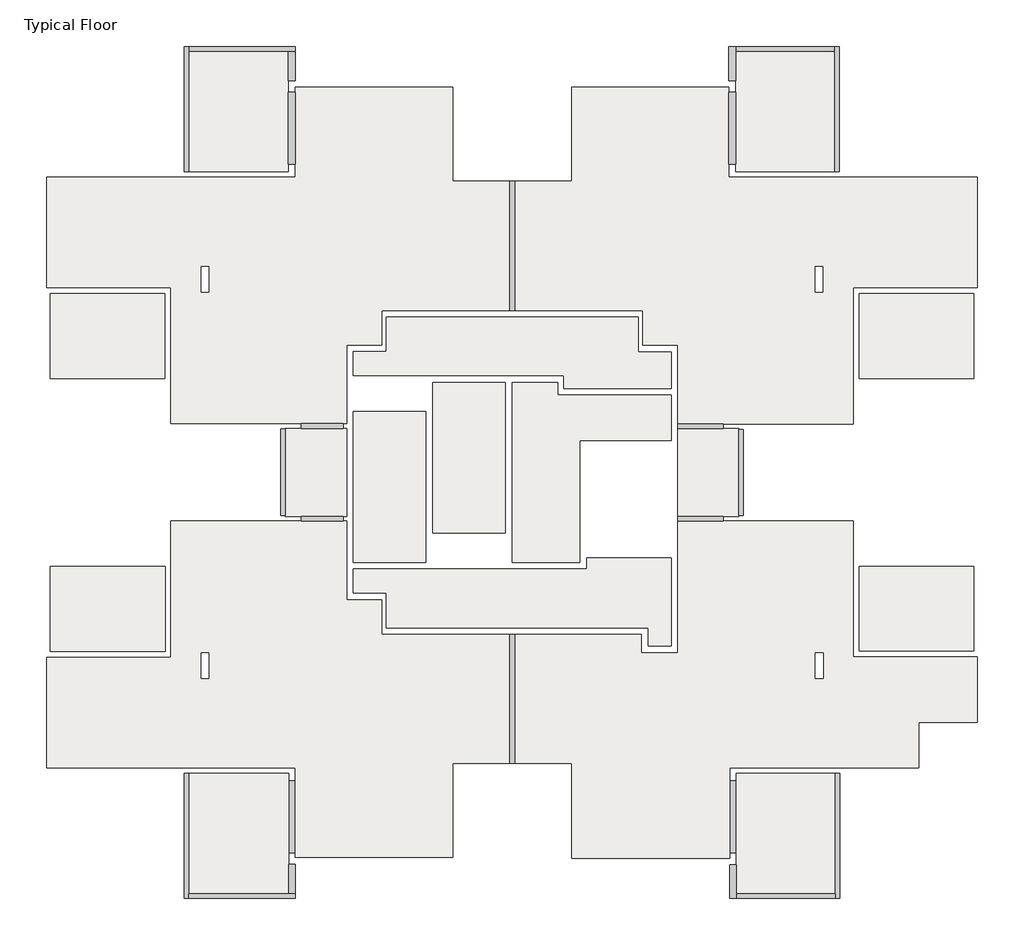
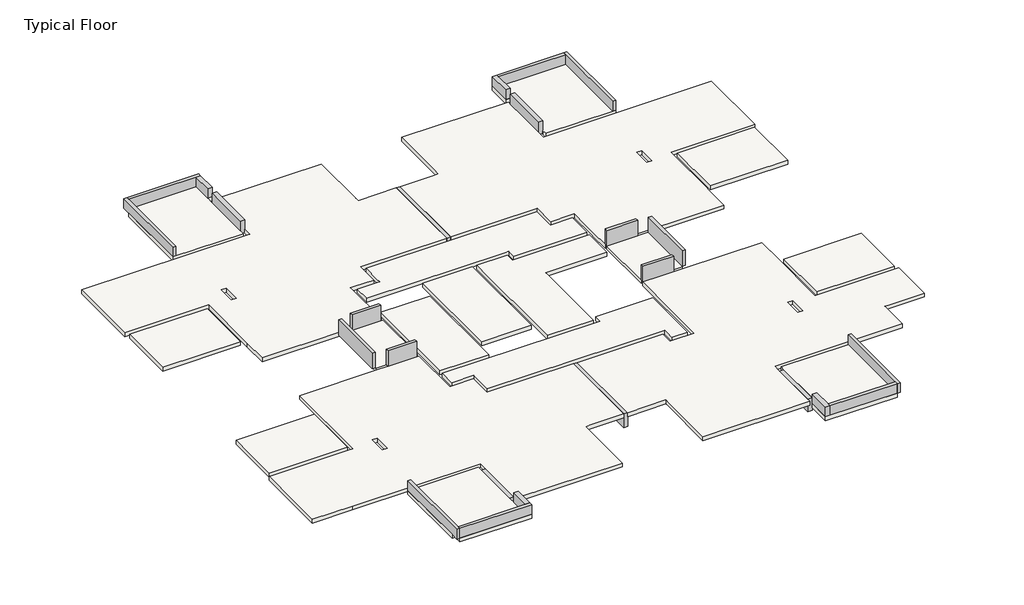
# One storey: 24 beams, 19 slabs.
"""IFC4 building model written with IfcOpenShell, lengths in millimetres."""

from ifc_helpers import new_model, si_unit, frame, origin, place, context, project, spatial, polyline, outline, extrude, faceted_brep, element, save

model = new_model("IFC4")

# Units and contexts
model_context = context("Model", 3, world=origin())
ifc_project = project(units=[si_unit("LENGTHUNIT", "METRE", prefix="MILLI")], contexts=[model_context])

# Site, building, storey
site = spatial("IfcSite", under=ifc_project)
building = spatial("IfcBuilding", under=site)
storey = spatial("IfcBuildingStorey", under=building, Name="Typical Floor", Elevation=3070.0)

# Beams
placement = place(None, origin())
element("IfcBeam", 1, ObjectType="Concrete Rectengular Beam : 15/50", at=placement, inside=storey, context=model_context, shape_type="Brep", body=[
    faceted_brep([(-14463.9862657, -10993.4504981, 3570.0), (-14313.9862657, -10993.4504981, 3570.0), (-14313.9862657, -10993.4504981, 3070.0), (-14463.9862657, -10993.4504981, 3070.0), (-14463.9862657, -15120.0113915, 3570.0), (-14313.9862657, -15120.0113915, 3570.0), (-14313.9862657, -14970.0113915, 3570.0), (-14313.9862657, -15120.0113915, 3070.0), (-14313.9862657, -14970.0113915, 3070.0), (-14313.9862657, -14720.0113915, 3070.0), (-14463.9862657, -15120.0113915, 3070.0), (-14463.9862657, -14720.0113915, 3070.0)], [[[0, 1, 2, 3]], [[1, 0, 4, 5, 6]], [[2, 1, 6, 5, 7, 8, 9]], [[3, 2, 9, 8, 7, 10, 11]], [[0, 3, 11, 10, 4]], [[5, 4, 10, 7]]]),
])
element("IfcBeam", 2, ObjectType="Concrete Rectengular Beam : 15/50", at=placement, inside=storey, context=model_context, shape_type="Brep", body=[
    faceted_brep([(-10809.6404044, -15120.0113915, 3570.0), (-10809.6404044, -14970.0113915, 3570.0), (-11029.6404044, -14970.0113915, 3570.0), (-14313.9862657, -14970.0113915, 3570.0), (-14313.9862657, -15120.0113915, 3570.0), (-10809.6404044, -15120.0113915, 3070.0), (-14313.9862657, -15120.0113915, 3070.0), (-10809.6404044, -14970.0113915, 3070.0), (-14313.9862657, -14970.0113915, 3070.0), (-11029.6404044, -14970.0113915, 3070.0)], [[[0, 1, 2, 3, 4]], [[5, 0, 4, 6]], [[7, 5, 6, 8, 9]], [[1, 7, 9, 8, 3, 2]], [[1, 0, 5, 7]], [[4, 3, 8, 6]]]),
])
element("IfcBeam", 3, ObjectType="Concrete Rectengular Beam : 15/50", at=placement, inside=storey, context=model_context, shape_type="Brep", body=[
    faceted_brep([(7011.4479352, -10993.4467583, 3570.0), (7161.4479352, -10993.4467583, 3570.0), (7161.4479352, -10993.4467583, 3070.0), (7011.4479352, -10993.4467583, 3070.0), (7011.4479352, -14970.0113915, 3570.0), (7011.4479352, -15120.0113915, 3570.0), (7161.4479352, -15120.0113915, 3570.0), (7011.4479352, -14720.0113915, 3070.0), (7011.4479352, -14970.0113915, 3070.0), (7011.4479352, -15120.0113915, 3070.0), (7161.4479352, -14720.0113915, 3070.0), (7161.4479352, -15120.0113915, 3070.0)], [[[0, 1, 2, 3]], [[1, 0, 4, 5, 6]], [[0, 3, 7, 8, 9, 5, 4]], [[3, 2, 10, 11, 9, 8, 7]], [[2, 1, 6, 11, 10]], [[6, 5, 9, 11]]]),
])
element("IfcBeam", 4, ObjectType="Concrete Rectengular Beam : 15/50", at=placement, inside=storey, context=model_context, shape_type="SweptSolid", body=[
    extrude(outline(polyline([(3739.0676082, -15120.0113915), (3739.0676082, -14970.0113915), (7011.4479352, -14970.0113915), (7011.4479352, -15120.0113915), (3739.0676082, -15120.0113915)])), frame((0.0, 0.0, 3070.0), z_axis=(0.0, 0.0, 1.0), x_axis=(1.0, 0.0, 0.0)), (0.0, 0.0, 1.0), 500.0),
])
element("IfcBeam", 5, ObjectType="Concrete Rectengular Beam : 15/50", at=placement, inside=storey, context=model_context, shape_type="Brep", body=[
    faceted_brep([(-14317.8223989, 8871.9475174, 3570.0), (-14467.8223989, 8871.9475174, 3570.0), (-14467.8223989, 8871.9475174, 3070.0), (-14317.8223989, 8871.9475174, 3070.0), (-14317.8223989, 12848.5060921, 3570.0), (-14317.8223989, 12998.5060921, 3570.0), (-14467.8223989, 12998.5060921, 3570.0), (-14317.8223989, 12598.5060921, 3070.0), (-14317.8223989, 12848.5060921, 3070.0), (-14317.8223989, 12998.5060921, 3070.0), (-14467.8223989, 12598.5060921, 3070.0), (-14467.8223989, 12998.5060921, 3070.0)], [[[0, 1, 2, 3]], [[1, 0, 4, 5, 6]], [[0, 3, 7, 8, 9, 5, 4]], [[3, 2, 10, 11, 9, 8, 7]], [[2, 1, 6, 11, 10]], [[6, 5, 9, 11]]]),
])
element("IfcBeam", 6, ObjectType="Concrete Rectengular Beam : 15/50", at=placement, inside=storey, context=model_context, shape_type="Brep", body=[
    faceted_brep([(-10813.4765376, 12848.5060921, 3570.0), (-10813.4765376, 12998.5060921, 3570.0), (-14317.8223989, 12998.5060921, 3570.0), (-14317.8223989, 12848.5060921, 3570.0), (-11033.4765376, 12848.5060921, 3570.0), (-10813.4765376, 12998.5060921, 3070.0), (-14317.8223989, 12998.5060921, 3070.0), (-10813.4765376, 12848.5060921, 3070.0), (-11033.4765376, 12848.5060921, 3070.0), (-14317.8223989, 12848.5060921, 3070.0)], [[[0, 1, 2, 3, 4]], [[1, 5, 6, 2]], [[5, 7, 8, 9, 6]], [[7, 0, 4, 3, 9, 8]], [[3, 2, 6, 9]], [[1, 0, 7, 5]]]),
])
element("IfcBeam", 7, ObjectType="Concrete Rectengular Beam : 15/50", at=placement, inside=storey, context=model_context, shape_type="Brep", body=[
    faceted_brep([(7142.0982792, 8871.9429548, 3570.0), (6992.0982792, 8871.9429548, 3570.0), (6992.0982792, 8871.9429548, 3070.0), (7142.0982792, 8871.9429548, 3070.0), (7142.0982792, 12998.507588, 3570.0), (6992.0982792, 12998.507588, 3570.0), (6992.0982792, 12848.507588, 3570.0), (6992.0982792, 12998.507588, 3070.0), (6992.0982792, 12848.507588, 3070.0), (6992.0982792, 12598.507588, 3070.0), (7142.0982792, 12998.507588, 3070.0), (7142.0982792, 12598.507588, 3070.0)], [[[0, 1, 2, 3]], [[1, 0, 4, 5, 6]], [[2, 1, 6, 5, 7, 8, 9]], [[3, 2, 9, 8, 7, 10, 11]], [[0, 3, 11, 10, 4]], [[5, 4, 10, 7]]]),
])
element("IfcBeam", 8, ObjectType="Concrete Rectengular Beam : 15/50", at=placement, inside=storey, context=model_context, shape_type="SweptSolid", body=[
    extrude(outline(polyline([(3719.7179522, 12848.507588), (3719.7179522, 12998.507588), (6992.0982792, 12998.507588), (6992.0982792, 12848.507588), (3719.7179522, 12848.507588)])), frame((0.0, 0.0, 3070.0), z_axis=(0.0, 0.0, 1.0), x_axis=(1.0, 0.0, 0.0)), (0.0, 0.0, 1.0), 500.0),
])
element("IfcBeam", 9, ObjectType="Concrete Rectengular Beam : 15/80", at=placement, inside=storey, context=model_context, shape_type="Brep", body=[
    faceted_brep([(-9219.5481077, -2506.5516458, 3870.0), (-9219.5481077, -2656.5516458, 3870.0), (-9219.5481077, -2656.5516458, 3070.0), (-9219.5481077, -2655.7878227, 3070.0), (-9219.5481077, -2506.5516458, 3070.0), (-10610.0280472, -2506.5516458, 3870.0), (-10610.0280472, -2506.5516458, 3070.0), (-10610.0280472, -2655.7878227, 3070.0), (-10610.0280472, -2656.5516458, 3070.0), (-10610.0280472, -2656.5516458, 3870.0)], [[[0, 1, 2, 3, 4]], [[5, 6, 7, 8, 9]], [[1, 0, 5, 9]], [[2, 1, 9, 8]], [[4, 3, 2, 8, 7, 6]], [[0, 4, 6, 5]]]),
])
element("IfcBeam", 10, ObjectType="Concrete Rectengular Beam : 15/80", at=placement, inside=storey, context=model_context, shape_type="Brep", body=[
    faceted_brep([(-9219.5481077, 546.2654793, 3870.0), (-9219.5481077, 396.2654793, 3870.0), (-9219.5481077, 396.2654793, 3070.0), (-9219.5481077, 396.7654793, 3070.0), (-9219.5481077, 546.2654793, 3070.0), (-10610.0280472, 546.2654793, 3870.0), (-10610.0280472, 546.2654793, 3070.0), (-10610.0280472, 396.7654793, 3070.0), (-10610.0280472, 396.2654793, 3070.0), (-10610.0280472, 396.2654793, 3870.0)], [[[0, 1, 2, 3, 4]], [[5, 6, 7, 8, 9]], [[1, 0, 5, 9]], [[2, 1, 9, 8]], [[4, 3, 2, 8, 7, 6]], [[0, 4, 6, 5]]]),
])
element("IfcBeam", 11, ObjectType="Concrete Rectengular Beam : 15/80", at=placement, inside=storey, context=model_context, shape_type="SweptSolid", body=[
    extrude(outline(polyline([(1809.3005209, -2656.5516458), (1809.3005209, -2506.5516458), (3307.48852, -2506.5516458), (3307.48852, -2656.5516458), (1809.3005209, -2656.5516458)])), frame((0.0, 0.0, 3070.0), z_axis=(0.0, 0.0, 1.0), x_axis=(1.0, 0.0, 0.0)), (0.0, 0.0, 1.0), 800.0),
])
element("IfcBeam", 12, ObjectType="Concrete Rectengular Beam : 15/80", at=placement, inside=storey, context=model_context, shape_type="SweptSolid", body=[
    extrude(outline(polyline([(1809.3005209, 390.6860076), (1809.3005209, 540.6860076), (3307.48852, 540.6860076), (3307.48852, 390.6860076), (1809.3005209, 390.6860076)])), frame((0.0, 0.0, 3070.0), z_axis=(0.0, 0.0, 1.0), x_axis=(1.0, 0.0, 0.0)), (0.0, 0.0, 1.0), 800.0),
])
element("IfcBeam", 13, ObjectType="Concrete Rectengular Beam : 15/80", at=placement, inside=storey, context=model_context, shape_type="SweptSolid", body=[
    extrude(outline(polyline([(3822.84243, 360.6860076), (3972.84243, 360.6860076), (3972.84243, -2476.2878227), (3822.84243, -2476.2878227), (3822.84243, 360.6860076)])), frame((0.0, 0.0, 3070.0), z_axis=(0.0, 0.0, 1.0), x_axis=(1.0, 0.0, 0.0)), (0.0, 0.0, 1.0), 800.0),
])
element("IfcBeam", 14, ObjectType="Concrete Rectengular Beam : 15/80", at=placement, inside=storey, context=model_context, shape_type="SweptSolid", body=[
    extrude(outline(polyline([(-11287.3486135, 366.7503763), (-11137.3486135, 366.7503763), (-11137.3486135, -2476.2878227), (-11287.3486135, -2476.2878227), (-11287.3486135, 366.7503763)])), frame((0.0, 0.0, 3070.0), z_axis=(0.0, 0.0, 1.0), x_axis=(1.0, 0.0, 0.0)), (0.0, 0.0, 1.0), 800.0),
])
element("IfcBeam", 15, ObjectType="Concrete Rectengular Beam : 20/70", at=placement, inside=storey, context=model_context, shape_type="Brep", body=[
    faceted_brep([(-3553.3678079, 8548.0720008, 3070.0), (-3753.3678079, 8548.0720008, 3070.0), (-3753.3678079, 4289.1186218, 3070.0), (-3553.3678079, 4289.1186218, 3070.0), (-3753.3678079, 8548.0720008, 2870.0), (-3753.3678079, 8548.0720008, 2370.0), (-3753.3678079, 4289.1186218, 2370.0), (-3753.3678079, 4289.1186218, 2870.0), (-3553.3678079, 8548.0720008, 2370.0), (-3553.3678079, 4289.1186218, 2370.0), (-3553.3678079, 8548.0720008, 2870.0), (-3553.3678079, 4289.1186218, 2870.0)], [[[0, 1, 2, 3]], [[1, 4, 5, 6, 7, 2]], [[5, 8, 9, 6]], [[8, 10, 0, 3, 11, 9]], [[1, 0, 10, 8, 5, 4]], [[3, 2, 7, 6, 9, 11]]]),
])
element("IfcBeam", 16, ObjectType="Concrete Rectengular Beam : 20/70", at=placement, inside=storey, context=model_context, shape_type="Brep", body=[
    faceted_brep([(-3553.3678079, -6410.6239212, 3070.0), (-3748.3678079, -6410.6239212, 3070.0), (-3748.3678079, -10669.5773003, 3070.0), (-3553.3678079, -10669.5773003, 3070.0), (-3753.3678079, -10669.5773003, 2870.0), (-3753.3678079, -6410.6239212, 2870.0), (-3753.3678079, -6410.6239212, 2370.0), (-3753.3678079, -10669.5773003, 2370.0), (-3553.3678079, -6410.6239212, 2370.0), (-3553.3678079, -10669.5773003, 2370.0), (-3553.3678079, -6410.6239212, 2870.0), (-3553.3678079, -10669.5773003, 2870.0), (-3748.3678079, -10669.5773003, 2870.0), (-3748.3678079, -6410.6239212, 2870.0)], [[[0, 1, 2, 3]], [[4, 5, 6, 7]], [[6, 8, 9, 7]], [[8, 10, 0, 3, 11, 9]], [[12, 13, 5, 4]], [[13, 12, 2, 1]], [[1, 0, 10, 8, 6, 5, 13]], [[3, 2, 12, 4, 7, 9, 11]]]),
])
element("IfcBeam", 17, ObjectType="Concrete Rectengular Beam : 22/50", at=placement, inside=storey, context=model_context, shape_type="Brep", body=[
    faceted_brep([(3739.0676082, -14009.5773003, 3570.0), (3739.0676082, -14009.5773003, 3070.0), (3519.0676082, -14009.5773003, 3070.0), (3519.0676082, -14009.5773003, 3570.0), (3519.0676082, -15120.0113915, 3570.0), (3739.0676082, -15120.0113915, 3570.0), (3739.0676082, -14970.0113915, 3570.0), (3519.0676082, -15120.0113915, 3070.0), (3739.0676082, -14970.0113915, 3070.0), (3739.0676082, -15120.0113915, 3070.0)], [[[0, 1, 2, 3]], [[0, 3, 4, 5, 6]], [[3, 2, 7, 4]], [[2, 1, 8, 9, 7]], [[1, 0, 6, 5, 9, 8]], [[5, 4, 7, 9]]]),
])
element("IfcBeam", 18, ObjectType="Concrete Rectengular Beam : 22/50", at=placement, inside=storey, context=model_context, shape_type="SweptSolid", body=[
    extrude(outline(polyline([(-11029.6404044, -13992.0681688), (-10809.6404044, -13992.0681688), (-10809.6404044, -14970.0113915), (-11029.6404044, -14970.0113915), (-11029.6404044, -13992.0681688)])), frame((0.0, 0.0, 3070.0), z_axis=(0.0, 0.0, 1.0), x_axis=(1.0, 0.0, 0.0)), (0.0, 0.0, 1.0), 500.0),
])
element("IfcBeam", 19, ObjectType="Concrete Rectengular Beam : 22/50", at=placement, inside=storey, context=model_context, shape_type="SweptSolid", body=[
    extrude(outline(polyline([(-10813.4765376, 11870.5628693), (-11033.4765376, 11870.5628693), (-11033.4765376, 12848.5060921), (-10813.4765376, 12848.5060921), (-10813.4765376, 11870.5628693)])), frame((0.0, 0.0, 3070.0), z_axis=(0.0, 0.0, 1.0), x_axis=(1.0, 0.0, 0.0)), (0.0, 0.0, 1.0), 500.0),
])
element("IfcBeam", 20, ObjectType="Concrete Rectengular Beam : 22/50", at=placement, inside=storey, context=model_context, shape_type="Brep", body=[
    faceted_brep([(3719.7179522, 11870.5628693, 3070.0), (3719.7179522, 11870.5628693, 3570.0), (3499.7179522, 11870.5628693, 3570.0), (3499.7179522, 11870.5628693, 3070.0), (3719.7179522, 12848.507588, 3570.0), (3719.7179522, 12998.507588, 3570.0), (3499.7179522, 12998.507588, 3570.0), (3499.7179522, 12998.507588, 3070.0), (3719.7179522, 12998.507588, 3070.0), (3719.7179522, 12848.507588, 3070.0)], [[[0, 1, 2, 3]], [[2, 1, 4, 5, 6]], [[3, 2, 6, 7]], [[0, 3, 7, 8, 9]], [[1, 0, 9, 8, 5, 4]], [[6, 5, 8, 7]]]),
])
element("IfcBeam", 21, ObjectType="Concrete Rectengular Beam : 22/65", at=placement, inside=storey, context=model_context, shape_type="Brep", body=[
    faceted_brep([(-11033.4765376, 11490.5628693, 3570.0), (-10813.4765376, 11490.5628693, 3570.0), (-10813.4765376, 11490.5628693, 3070.0), (-10813.4765376, 11490.5628693, 2920.0), (-11033.4765376, 11490.5628693, 2920.0), (-11033.4765376, 11490.5628693, 3070.0), (-11033.4765376, 9111.6813756, 2920.0), (-10813.4765376, 9111.6813756, 2920.0), (-10813.4765376, 9111.6813756, 3070.0), (-10813.4765376, 9111.6813756, 3570.0), (-11033.4765376, 9111.6813756, 3570.0), (-11033.4765376, 9111.6813756, 3070.0), (-11033.4765376, 9111.9475174, 2920.0)], [[[0, 1, 2, 3, 4, 5]], [[6, 7, 8, 9, 10, 11]], [[1, 0, 10, 9]], [[1, 9, 8, 7, 3, 2]], [[4, 3, 7, 6, 12]], [[10, 0, 5, 4, 12, 6, 11]]]),
])
element("IfcBeam", 22, ObjectType="Concrete Rectengular Beam : 22/65", at=placement, inside=storey, context=model_context, shape_type="Brep", body=[
    faceted_brep([(3719.7179522, 9111.9429548, 3570.0), (3499.7179522, 9111.9429548, 3570.0), (3499.7179522, 9111.9429548, 3070.0), (3499.7179522, 9111.9429548, 2920.0), (3719.7179522, 9111.9429548, 2920.0), (3719.7179522, 9111.9429548, 3070.0), (3719.7179522, 11490.5628693, 2920.0), (3499.7179522, 11490.5628693, 2920.0), (3499.7179522, 11490.5628693, 3070.0), (3499.7179522, 11490.5628693, 3570.0), (3719.7179522, 11490.5628693, 3570.0), (3719.7179522, 11490.5628693, 3070.0)], [[[0, 1, 2, 3, 4, 5]], [[6, 7, 8, 9, 10, 11]], [[1, 0, 10, 9]], [[1, 9, 8, 7, 3, 2]], [[4, 3, 7, 6]], [[10, 0, 5, 4, 6, 11]]]),
])
element("IfcBeam", 23, ObjectType="Concrete Rectengular Beam : 22/65", at=placement, inside=storey, context=model_context, shape_type="SweptSolid", body=[
    extrude(outline(polyline([(-10809.6404044, -13620.3281962), (-11029.6404044, -13620.3281962), (-11029.6404044, -11233.4504981), (-10809.6404044, -11233.4504981), (-10809.6404044, -13620.3281962)])), frame((0.0, 0.0, 2420.0), z_axis=(0.0, 0.0, 1.0), x_axis=(1.0, 0.0, 0.0)), (0.0, 0.0, 1.0), 650.0),
])
element("IfcBeam", 24, ObjectType="Concrete Rectengular Beam : 22/65", at=placement, inside=storey, context=model_context, shape_type="Brep", body=[
    faceted_brep([(3739.0676082, -13619.5773003, 3070.0), (3519.0676082, -13619.5773003, 3070.0), (3519.0676082, -13619.5773003, 2870.0), (3519.0676082, -13619.5773003, 2420.0), (3739.0676082, -13619.5773003, 2420.0), (3739.0676082, -13619.5773003, 2870.0), (3739.0676082, -11233.4467583, 2420.0), (3519.0676082, -11233.4467583, 2420.0), (3519.0676082, -11233.4467583, 2870.0), (3519.0676082, -11233.4467583, 3070.0), (3739.0676082, -11233.4467583, 3070.0), (3739.0676082, -11233.4467583, 2870.0)], [[[0, 1, 2, 3, 4, 5]], [[6, 7, 8, 9, 10, 11]], [[1, 0, 10, 9]], [[1, 9, 8, 7, 3, 2]], [[4, 3, 7, 6]], [[10, 0, 5, 4, 6, 11]]]),
])

# Slabs
element("IfcSlab", 25, ObjectType="15", at=placement, inside=storey, context=model_context, shape_type="Brep", body=[
    faceted_brep([(-9111.0923752, -2506.5516458, 2920.0), (-11137.3486135, -2506.5516458, 2920.0), (-11137.3486135, 396.2654793, 2920.0), (-10610.0280472, 396.2654793, 2920.0), (-10610.0280472, 396.7654793, 2920.0), (-9219.5481077, 396.7654793, 2920.0), (-9219.5481077, 396.2654793, 2920.0), (-9111.0923752, 396.2654793, 2920.0), (-11137.3486135, -2506.5516458, 3070.0), (-10610.0280472, -2506.5516458, 3070.0), (-9219.5481077, -2506.5516458, 3070.0), (-9111.0923752, -2506.5516458, 3070.0), (-9111.0923752, 396.2654793, 3070.0), (-9219.5481077, 396.2654793, 3070.0), (-9219.5481077, 396.7654793, 3070.0), (-10610.0280472, 396.7654793, 3070.0), (-10610.0280472, 396.2654793, 3070.0), (-11137.3486135, 396.2654793, 3070.0), (-11137.3486135, 366.7503763, 3070.0), (-11137.3486135, -2476.2878227, 3070.0)], [[[0, 1, 2, 3, 4, 5, 6, 7]], [[8, 9, 10, 11, 12, 13, 14, 15, 16, 17, 18, 19]], [[14, 5, 4, 15]], [[11, 0, 7, 12]], [[1, 0, 11, 10, 9, 8]], [[1, 8, 19, 18, 17, 2]], [[6, 13, 12, 7]], [[13, 6, 5, 14]], [[16, 3, 2, 17]], [[3, 16, 15, 4]]]),
])
element("IfcSlab", 26, ObjectType="15", at=placement, inside=storey, context=model_context, shape_type="Brep", body=[
    faceted_brep([(3822.84243, 390.6860076, 2920.0), (3822.84243, -2506.5516458, 2920.0), (1809.3005209, -2506.5516458, 2920.0), (1809.3005209, 390.6860076, 2920.0), (3822.84243, 390.6860076, 3070.0), (3307.48852, 390.6860076, 3070.0), (1809.3005209, 390.6860076, 3070.0), (1809.3005209, -2506.5516458, 3070.0), (3307.48852, -2506.5516458, 3070.0), (3822.84243, -2506.5516458, 3070.0), (3822.84243, -2476.2878227, 3070.0), (3822.84243, 360.6860076, 3070.0)], [[[0, 1, 2, 3]], [[4, 5, 6, 7, 8, 9, 10, 11]], [[1, 0, 4, 11, 10, 9]], [[2, 1, 9, 8, 7]], [[3, 2, 7, 6]], [[0, 3, 6, 5, 4]]]),
])
element("IfcSlab", 27, ObjectType="20", at=placement, inside=storey, context=model_context, shape_type="Brep", body=[
    faceted_brep([(-11029.6404044, -10993.4504981, 2870.0), (-11029.6404044, -11233.4504981, 2870.0), (-11029.6404044, -13620.3281962, 2870.0), (-11029.6404044, -13992.0681688, 2870.0), (-10809.6404044, -13992.0681688, 2870.0), (-10809.6404044, -15120.0113915, 2870.0), (-14313.9862657, -15120.0113915, 2870.0), (-14313.9862657, -14720.0113915, 2870.0), (-14463.9862657, -14720.0113915, 2870.0), (-14463.9862657, -10993.4504981, 2870.0), (-14313.9862657, -10993.4504981, 2870.0), (-11029.6404044, -11233.4504981, 3070.0), (-11029.6404044, -10993.4504981, 3070.0), (-14313.9862657, -10993.4504981, 3070.0), (-14463.9862657, -10993.4504981, 3070.0), (-14463.9862657, -14720.0113915, 3070.0), (-14313.9862657, -14720.0113915, 3070.0), (-14313.9862657, -14970.0113915, 3070.0), (-14313.9862657, -15120.0113915, 3070.0), (-10809.6404044, -15120.0113915, 3070.0), (-10809.6404044, -14970.0113915, 3070.0), (-10809.6404044, -13992.0681688, 3070.0), (-11029.6404044, -13992.0681688, 3070.0), (-11029.6404044, -13620.3281962, 3070.0)], [[[0, 1, 2, 3, 4, 5, 6, 7, 8, 9, 10]], [[11, 12, 13, 14, 15, 16, 17, 18, 19, 20, 21, 22, 23]], [[1, 0, 12, 11]], [[2, 1, 11, 23]], [[3, 2, 23, 22]], [[4, 3, 22, 21]], [[5, 4, 21, 20, 19]], [[5, 19, 18, 6]], [[14, 9, 8, 15]], [[10, 9, 14, 13]], [[0, 10, 13, 12]], [[16, 7, 6, 18, 17]], [[7, 16, 15, 8]]]),
])
element("IfcSlab", 28, ObjectType="20", at=placement, inside=storey, context=model_context, shape_type="Brep", body=[
    faceted_brep([(3519.0676082, -15120.0113915, 2870.0), (3519.0676082, -14009.5773003, 2870.0), (3739.0676082, -14009.5773003, 2870.0), (3739.0676082, -13619.5773003, 2870.0), (3739.0676082, -11233.4467583, 2870.0), (3739.0676082, -10993.4467583, 2870.0), (7161.4479352, -10993.4467583, 2870.0), (7161.4479352, -14720.0113915, 2870.0), (7011.4479352, -14720.0113915, 2870.0), (7011.4479352, -15120.0113915, 2870.0), (3519.0676082, -14009.5773003, 3070.0), (3519.0676082, -15120.0113915, 3070.0), (3739.0676082, -15120.0113915, 3070.0), (7011.4479352, -15120.0113915, 3070.0), (7011.4479352, -14970.0113915, 3070.0), (7011.4479352, -14720.0113915, 3070.0), (7161.4479352, -14720.0113915, 3070.0), (7161.4479352, -10993.4467583, 3070.0), (7011.4479352, -10993.4467583, 3070.0), (3739.0676082, -10993.4467583, 3070.0), (3739.0676082, -11233.4467583, 3070.0), (3739.0676082, -13619.5773003, 3070.0), (3739.0676082, -14009.5773003, 3070.0)], [[[0, 1, 2, 3, 4, 5, 6, 7, 8, 9]], [[10, 11, 12, 13, 14, 15, 16, 17, 18, 19, 20, 21, 22]], [[6, 17, 16, 7]], [[11, 0, 9, 13, 12]], [[1, 0, 11, 10]], [[2, 1, 10, 22]], [[3, 2, 22, 21]], [[4, 3, 21, 20]], [[5, 4, 20, 19]], [[6, 5, 19, 18, 17]], [[8, 15, 14, 13, 9]], [[15, 8, 7, 16]]]),
])
element("IfcSlab", 29, ObjectType="20", at=placement, inside=storey, context=model_context, shape_type="Brep", body=[
    faceted_brep([(-11033.4765376, 11870.565188, 2870.0), (-11033.4765376, 11498.8252154, 2870.0), (-11033.4765376, 11490.5628693, 2870.0), (-11033.4765376, 9111.9475174, 2870.0), (-11033.4765376, 9111.6813756, 2870.0), (-11033.4765376, 8871.6813756, 2870.0), (-14467.8223989, 8871.6813756, 2870.0), (-14467.8223989, 12598.5060921, 2870.0), (-14317.8223989, 12598.5060921, 2870.0), (-14317.8223989, 12998.5084108, 2870.0), (-10813.4765376, 12998.5084108, 2870.0), (-10813.4765376, 11870.565188, 2870.0), (-11033.4765376, 11498.8252154, 3070.0), (-11033.4765376, 11870.565188, 3070.0), (-10813.4765376, 11870.565188, 3070.0), (-10813.4765376, 12848.5060921, 3070.0), (-10813.4765376, 12998.5084108, 3070.0), (-14317.8223989, 12998.5084108, 3070.0), (-14317.8223989, 12848.5060921, 3070.0), (-14317.8223989, 12598.5060921, 3070.0), (-14467.8223989, 12598.5060921, 3070.0), (-14467.8223989, 8871.9475174, 3070.0), (-14467.8223989, 8871.6813756, 3070.0), (-11033.4765376, 8871.6813756, 3070.0), (-11033.4765376, 9111.6813756, 3070.0), (-11033.4765376, 9111.9475174, 3070.0), (-11033.4765376, 11490.5628693, 3070.0)], [[[0, 1, 2, 3, 4, 5, 6, 7, 8, 9, 10, 11]], [[12, 13, 14, 15, 16, 17, 18, 19, 20, 21, 22, 23, 24, 25, 26]], [[3, 25, 24, 23, 5, 4]], [[1, 12, 26, 25, 3, 2]], [[1, 0, 13, 12]], [[0, 11, 14, 13]], [[11, 10, 16, 15, 14]], [[16, 10, 9, 17]], [[20, 7, 6, 22, 21]], [[8, 19, 18, 17, 9]], [[19, 8, 7, 20]], [[6, 5, 23, 22]]]),
])
element("IfcSlab", 30, ObjectType="20", at=placement, inside=storey, context=model_context, shape_type="Brep", body=[
    faceted_brep([(3499.7179522, 11870.5628693, 2870.0), (3499.7179522, 12998.507588, 2870.0), (6992.0982792, 12998.507588, 2870.0), (6992.0982792, 12598.507588, 2870.0), (7142.0982792, 12598.507588, 2870.0), (7142.0982792, 8871.9429548, 2870.0), (3719.7179522, 8871.9429548, 2870.0), (3719.7179522, 9111.9429548, 2870.0), (3719.7179522, 11490.5628693, 2870.0), (3719.7179522, 11498.0734968, 2870.0), (3719.7179522, 11870.5628693, 2870.0), (3499.7179522, 12998.507588, 3070.0), (3499.7179522, 11870.5628693, 3070.0), (3719.7179522, 11870.5628693, 3070.0), (3719.7179522, 11498.0734968, 3070.0), (3719.7179522, 11490.5628693, 3070.0), (3719.7179522, 9111.9429548, 3070.0), (3719.7179522, 8871.9429548, 3070.0), (6992.0982792, 8871.9429548, 3070.0), (7142.0982792, 8871.9429548, 3070.0), (7142.0982792, 12598.507588, 3070.0), (6992.0982792, 12598.507588, 3070.0), (6992.0982792, 12848.507588, 3070.0), (6992.0982792, 12998.507588, 3070.0), (3719.7179522, 12998.507588, 3070.0)], [[[0, 1, 2, 3, 4, 5, 6, 7, 8, 9, 10]], [[11, 12, 13, 14, 15, 16, 17, 18, 19, 20, 21, 22, 23, 24]], [[19, 5, 4, 20]], [[1, 11, 24, 23, 2]], [[1, 0, 12, 11]], [[0, 10, 13, 12]], [[10, 9, 14, 13]], [[7, 16, 15, 14, 9, 8]], [[7, 6, 17, 16]], [[6, 5, 19, 18, 17]], [[21, 3, 2, 23, 22]], [[3, 21, 20, 4]]]),
])
element("IfcSlab", 31, ObjectType="20", at=placement, inside=storey, context=model_context, shape_type="SweptSolid", body=[
    extrude(outline(polyline([(-15113.1120804, 4845.3187304), (-15113.1120804, 2043.8819255), (-18893.0086039, 2043.8819255), (-18893.0086039, 4845.3187304), (-15113.1120804, 4845.3187304)])), frame((0.0, 0.0, 2870.0), z_axis=(0.0, 0.0, 1.0), x_axis=(1.0, 0.0, 0.0)), (0.0, 0.0, 1.0), 200.0),
])
element("IfcSlab", 32, ObjectType="20", at=placement, inside=storey, context=model_context, shape_type="SweptSolid", body=[
    extrude(outline(polyline([(11579.3119283, 4841.1223427), (11579.3119283, 2043.8824455), (7802.84243, 2043.8824455), (7802.84243, 4841.1223427), (11579.3119283, 4841.1223427)])), frame((0.0, 0.0, 2870.0), z_axis=(0.0, 0.0, 1.0), x_axis=(1.0, 0.0, 0.0)), (0.0, 0.0, 1.0), 200.0),
])
element("IfcSlab", 33, ObjectType="20", at=placement, inside=storey, context=model_context, shape_type="SweptSolid", body=[
    extrude(outline(polyline([(-15093.3730612, -4166.1341463), (-15093.3730612, -6966.8226087), (-18893.0716357, -6966.8226087), (-18893.0716357, -4166.1341463), (-15093.3730612, -4166.1341463)])), frame((0.0, 0.0, 2870.0), z_axis=(0.0, 0.0, 1.0), x_axis=(1.0, 0.0, 0.0)), (0.0, 0.0, 1.0), 200.0),
])
element("IfcSlab", 34, ObjectType="20", at=placement, inside=storey, context=model_context, shape_type="SweptSolid", body=[
    extrude(outline(polyline([(11579.3119283, -4166.1341463), (11579.3119283, -6953.7627402), (7800.4432059, -6953.7627402), (7800.4432059, -4166.1341463), (11579.3119283, -4166.1341463)])), frame((0.0, 0.0, 2870.0), z_axis=(0.0, 0.0, 1.0), x_axis=(1.0, 0.0, 0.0)), (0.0, 0.0, 1.0), 200.0),
])
element("IfcSlab", 35, ObjectType="20", at=placement, inside=storey, context=model_context, shape_type="Brep", body=[
    faceted_brep([(7600.4432059, -7153.7627402, 2870.0), (11698.5007748, -7153.7627402, 2870.0), (11698.5007748, -9313.7627402, 2870.0), (9937.2529005, -9313.7627402, 2870.0), (9757.2529005, -9313.7627402, 2870.0), (9757.2529005, -10813.4467583, 2870.0), (3739.0676082, -10813.4467583, 2870.0), (3519.0676082, -10813.4467583, 2870.0), (3519.0676082, -11233.4467583, 2870.0), (3519.0676082, -13619.5773003, 2870.0), (3519.0676082, -13789.5773003, 2870.0), (-1691.2080852, -13789.5773003, 2870.0), (-1691.2080852, -10849.5773003, 2870.0), (-1691.2080852, -10669.5773003, 2870.0), (-3553.3678079, -10669.5773003, 2870.0), (-3553.3678079, -6410.6239212, 2870.0), (610.3012935, -6410.6239212, 2870.0), (610.3012935, -7010.4989795, 2870.0), (830.3012935, -7010.4989795, 2870.0), (1809.3005209, -7010.4989795, 2870.0), (1809.3005209, -6790.4989795, 2870.0), (1809.3005209, -2656.5516458, 2870.0), (7600.4432059, -2656.5516458, 2870.0), (7600.4432059, -4041.1341463, 2870.0), (7600.4432059, -6953.7627402, 2870.0), (6603.8022343, -7860.4989795, 2870.0), (6603.8022343, -7010.4989795, 2870.0), (6353.8022343, -7010.4989795, 2870.0), (6353.8022343, -7860.4989795, 2870.0), (11698.5007748, -7153.7627402, 3070.0), (7600.4432059, -7153.7627402, 3070.0), (7600.4432059, -6953.7627402, 3070.0), (7600.4432059, -4041.1341463, 3070.0), (7600.4432059, -2656.5516458, 3070.0), (3822.84243, -2656.5516458, 3070.0), (3307.48852, -2656.5516458, 3070.0), (1809.3005209, -2656.5516458, 3070.0), (1809.3005209, -6790.4989795, 3070.0), (1809.3005209, -7010.4989795, 3070.0), (830.3012935, -7010.4989795, 3070.0), (610.3012935, -7010.4989795, 3070.0), (610.3012935, -6410.6239212, 3070.0), (-3553.3678079, -6410.6239212, 3070.0), (-3553.3678079, -10669.5773003, 3070.0), (-1691.2080852, -10669.5773003, 3070.0), (-1691.2080852, -10849.5773003, 3070.0), (-1691.2080852, -13789.5773003, 3070.0), (3519.0676082, -13789.5773003, 3070.0), (3519.0676082, -13619.5773003, 3070.0), (3519.0676082, -11233.4467583, 3070.0), (3519.0676082, -10813.4467583, 3070.0), (3739.0676082, -10813.4467583, 3070.0), (9757.2529005, -10813.4467583, 3070.0), (9757.2529005, -9313.7627402, 3070.0), (9937.2529005, -9313.7627402, 3070.0), (11698.5007748, -9313.7627402, 3070.0), (6603.8022343, -7010.4989795, 3070.0), (6603.8022343, -7860.4989795, 3070.0), (6353.8022343, -7860.4989795, 3070.0), (6353.8022343, -7010.4989795, 3070.0)], [[[0, 1, 2, 3, 4, 5, 6, 7, 8, 9, 10, 11, 12, 13, 14, 15, 16, 17, 18, 19, 20, 21, 22, 23, 24], [25, 26, 27, 28]], [[29, 30, 31, 32, 33, 34, 35, 36, 37, 38, 39, 40, 41, 42, 43, 44, 45, 46, 47, 48, 49, 50, 51, 52, 53, 54, 55], [56, 57, 58, 59]], [[30, 0, 24, 23, 22, 33, 32, 31]], [[1, 0, 30, 29]], [[2, 1, 29, 55]], [[2, 55, 54, 53, 4, 3]], [[5, 4, 53, 52]], [[5, 52, 51, 50, 7, 6]], [[7, 50, 49, 48, 47, 10, 9, 8]], [[11, 10, 47, 46]], [[11, 46, 45, 44, 13, 12]], [[14, 13, 44, 43]], [[15, 14, 43, 42]], [[16, 15, 42, 41]], [[17, 16, 41, 40]], [[17, 40, 39, 38, 19, 18]], [[19, 38, 37, 36, 21, 20]], [[22, 21, 36, 35, 34, 33]], [[25, 57, 56, 26]], [[57, 25, 28, 58]], [[58, 28, 27, 59]], [[59, 27, 26, 56]]]),
])
element("IfcSlab", 36, ObjectType="20", at=placement, inside=storey, context=model_context, shape_type="Brep", body=[
    faceted_brep([(-19012.7470995, -10813.4504981, 2870.0), (-19012.7470995, -7166.8226087, 2870.0), (-18893.0716357, -7166.8226087, 2870.0), (-15093.3730612, -7166.8226087, 2870.0), (-14913.3730612, -7166.8226087, 2870.0), (-14913.3730612, -2656.2878227, 2870.0), (-11137.3486135, -2656.2878227, 2870.0), (-11137.3486135, -2656.5516458, 2870.0), (-10610.0280472, -2656.5516458, 2870.0), (-10610.0280472, -2655.7878227, 2870.0), (-9219.5481077, -2655.7878227, 2870.0), (-9219.5481077, -2656.5516458, 2870.0), (-9111.0923752, -2656.5516458, 2870.0), (-9111.0923752, -5263.3286489, 2870.0), (-8891.0923752, -5263.3286489, 2870.0), (-7960.7109614, -5263.3286489, 2870.0), (-7960.7109614, -6190.6239212, 2870.0), (-7960.7109614, -6410.6239212, 2870.0), (-3753.3678079, -6410.6239212, 2870.0), (-3748.3678079, -6410.6239212, 2870.0), (-3748.3678079, -10669.5773003, 2870.0), (-3753.3678079, -10669.5773003, 2870.0), (-5431.3302453, -10669.5773003, 2870.0), (-5611.3302453, -10669.5773003, 2870.0), (-5611.3302453, -13772.0681688, 2870.0), (-10809.6404044, -13772.0681688, 2870.0), (-10809.6404044, -13620.3281962, 2870.0), (-10809.6404044, -11233.4504981, 2870.0), (-10809.6404044, -10813.4467583, 2870.0), (-11029.6404044, -10813.4467583, 2870.0), (-17063.9885163, -10813.4467583, 2870.0), (-13656.3416868, -7860.4989795, 2870.0), (-13656.3416868, -7010.4989795, 2870.0), (-13906.3416868, -7010.4989795, 2870.0), (-13906.3416868, -7860.4989795, 2870.0), (-19012.7470995, -7166.8226087, 3070.0), (-19012.7470995, -10813.4504981, 3070.0), (-17063.9885163, -10813.4504981, 3070.0), (-11029.6404044, -10813.4467583, 3070.0), (-10809.6404044, -10813.4467583, 3070.0), (-10809.6404044, -11233.4504981, 3070.0), (-10809.6404044, -13620.3281962, 3070.0), (-10809.6404044, -13772.0681688, 3070.0), (-5611.3302453, -13772.0681688, 3070.0), (-5611.3302453, -10669.5773003, 3070.0), (-5431.3302453, -10669.5773003, 3070.0), (-3748.3678079, -10669.5773003, 3070.0), (-3748.3678079, -6410.6239212, 3070.0), (-7960.7109614, -6410.6239212, 3070.0), (-7960.7109614, -6190.6239212, 3070.0), (-7960.7109614, -5263.3286489, 3070.0), (-8891.0923752, -5263.3286489, 3070.0), (-9111.0923752, -5263.3286489, 3070.0), (-9111.0923752, -2656.5516458, 3070.0), (-9219.5481077, -2656.5516458, 3070.0), (-9219.5481077, -2655.7878227, 3070.0), (-10610.0280472, -2655.7878227, 3070.0), (-10610.0280472, -2656.5516458, 3070.0), (-11137.3486135, -2656.5516458, 3070.0), (-11137.3486135, -2656.2878227, 3070.0), (-14913.3730612, -2656.2878227, 3070.0), (-14913.3730612, -7166.8226087, 3070.0), (-15093.3730612, -7166.8226087, 3070.0), (-18893.0716357, -7166.8226087, 3070.0), (-13656.3416868, -7010.4989795, 3070.0), (-13656.3416868, -7860.4989795, 3070.0), (-13906.3416868, -7860.4989795, 3070.0), (-13906.3416868, -7010.4989795, 3070.0)], [[[0, 1, 2, 3, 4, 5, 6, 7, 8, 9, 10, 11, 12, 13, 14, 15, 16, 17, 18, 19, 20, 21, 22, 23, 24, 25, 26, 27, 28, 29, 30], [31, 32, 33, 34]], [[35, 36, 37, 38, 39, 40, 41, 42, 43, 44, 45, 46, 47, 48, 49, 50, 51, 52, 53, 54, 55, 56, 57, 58, 59, 60, 61, 62, 63], [64, 65, 66, 67]], [[4, 61, 60, 5]], [[1, 35, 63, 62, 61, 4, 3, 2]], [[1, 0, 36, 35]], [[0, 30, 37, 36]], [[28, 39, 38, 37, 30, 29]], [[25, 42, 41, 40, 39, 28, 27, 26]], [[25, 24, 43, 42]], [[24, 23, 44, 43]], [[20, 46, 45, 44, 23, 22, 21]], [[20, 19, 47, 46]], [[19, 18, 17, 48, 47]], [[15, 50, 49, 48, 17, 16]], [[13, 52, 51, 50, 15, 14]], [[52, 13, 12, 53]], [[9, 56, 55, 10]], [[31, 65, 64, 32]], [[65, 31, 34, 66]], [[66, 34, 33, 67]], [[67, 33, 32, 64]], [[6, 5, 60, 59]], [[7, 58, 57, 8]], [[8, 57, 56, 9]], [[58, 7, 6, 59]], [[11, 54, 53, 12]], [[54, 11, 10, 55]]]),
])
element("IfcSlab", 37, ObjectType="20", at=placement, inside=storey, context=model_context, shape_type="Brep", body=[
    faceted_brep([(-1195.2062248, -4251.9774411, 2870.0), (-1195.2062248, -3884.0679171, 2870.0), (1589.3005209, -3884.0679171, 2870.0), (1589.3005209, -6790.4989795, 2870.0), (830.3012935, -6790.4989795, 2870.0), (830.3012935, -6190.6239212, 2870.0), (610.3012935, -6190.6239212, 2870.0), (-7810.7109614, -6190.6239212, 2870.0), (-7810.7109614, -5263.3286489, 2870.0), (-7810.7109614, -5043.3286489, 2870.0), (-8891.0923752, -5043.3286489, 2870.0), (-8891.0923752, -4251.9774411, 2870.0), (-1415.2062248, -4251.9774411, 2870.0), (-1195.2062248, -3884.0679171, 3070.0), (-1195.2062248, -4251.9774411, 3070.0), (-1415.2062248, -4251.9774411, 3070.0), (-8891.0923752, -4251.9774411, 3070.0), (-8891.0923752, -5043.3286489, 3070.0), (-7810.7109614, -5043.3286489, 3070.0), (-7810.7109614, -5263.3286489, 3070.0), (-7810.7109614, -6190.6239212, 3070.0), (610.3012935, -6190.6239212, 3070.0), (830.3012935, -6190.6239212, 3070.0), (830.3012935, -6790.4989795, 3070.0), (1589.3005209, -6790.4989795, 3070.0), (1589.3005209, -3884.0679171, 3070.0)], [[[0, 1, 2, 3, 4, 5, 6, 7, 8, 9, 10, 11, 12]], [[13, 14, 15, 16, 17, 18, 19, 20, 21, 22, 23, 24, 25]], [[1, 0, 14, 13]], [[2, 1, 13, 25]], [[3, 2, 25, 24]], [[4, 3, 24, 23]], [[5, 4, 23, 22]], [[5, 22, 21, 20, 7, 6]], [[7, 20, 19, 18, 9, 8]], [[10, 9, 18, 17]], [[11, 10, 17, 16]], [[11, 16, 15, 14, 0, 12]]]),
])
element("IfcSlab", 38, ObjectType="20", at=placement, inside=storey, context=model_context, shape_type="Brep", body=[
    faceted_brep([(-2155.2421674, 1914.3048342, 2870.0), (-2155.2421674, 1493.9448789, 2870.0), (-1955.2421674, 1493.9448789, 2870.0), (1589.3005209, 1493.9448789, 2870.0), (1589.3005209, -4.9895964, 2870.0), (-1415.2062248, -4.9895964, 2870.0), (-1415.2062248, -154.9895964, 2870.0), (-1415.2062248, -3664.0679171, 2870.0), (-1415.2062248, -4031.9774411, 2870.0), (-3653.0437953, -4031.9774411, 2870.0), (-3653.0437953, 1914.3048342, 2870.0), (-2155.2421674, 1493.9448789, 3070.0), (-2155.2421674, 1914.3048342, 3070.0), (-3653.0437953, 1914.3048342, 3070.0), (-3653.0437953, -4031.9774411, 3070.0), (-1415.2062248, -4031.9774411, 3070.0), (-1415.2062248, -3664.0679171, 3070.0), (-1415.2062248, -154.9895964, 3070.0), (-1415.2062248, -4.9895964, 3070.0), (1589.3005209, -4.9895964, 3070.0), (1589.3005209, 1493.9448789, 3070.0), (-1955.2421674, 1493.9448789, 3070.0)], [[[0, 1, 2, 3, 4, 5, 6, 7, 8, 9, 10]], [[11, 12, 13, 14, 15, 16, 17, 18, 19, 20, 21]], [[1, 0, 12, 11]], [[1, 11, 21, 20, 3, 2]], [[4, 3, 20, 19]], [[5, 4, 19, 18]], [[5, 18, 17, 16, 15, 8, 7, 6]], [[9, 8, 15, 14]], [[10, 9, 14, 13]], [[0, 10, 13, 12]]]),
])
element("IfcSlab", 39, ObjectType="20", at=placement, inside=storey, context=model_context, shape_type="SweptSolid", body=[
    extrude(outline(polyline([(-3873.0437953, 1914.3048342), (-3873.0437953, -3064.1974214), (-6278.4263718, -3064.1974214), (-6278.4263718, 1914.3048342), (-3873.0437953, 1914.3048342)])), frame((0.0, 0.0, 2870.0), z_axis=(0.0, 0.0, 1.0), x_axis=(1.0, 0.0, 0.0)), (0.0, 0.0, 1.0), 200.0),
])
element("IfcSlab", 40, ObjectType="20", at=placement, inside=storey, context=model_context, shape_type="SweptSolid", body=[
    extrude(outline(polyline([(-6498.4263718, 942.6898033), (-6498.4263718, -4031.9774411), (-8891.0923752, -4031.9774411), (-8891.0923752, 942.6898033), (-6498.4263718, 942.6898033)])), frame((0.0, 0.0, 2870.0), z_axis=(0.0, 0.0, 1.0), x_axis=(1.0, 0.0, 0.0)), (0.0, 0.0, 1.0), 200.0),
])
element("IfcSlab", 41, ObjectType="20", at=placement, inside=storey, context=model_context, shape_type="Brep", body=[
    faceted_brep([(508.1725561, 2917.988413, 2870.0), (1589.3005209, 2917.988413, 2870.0), (1589.3005209, 1713.9448789, 2870.0), (-1955.2421674, 1713.9448789, 2870.0), (-1955.2421674, 2134.3048342, 2870.0), (-2155.2421674, 2134.3048342, 2870.0), (-8891.0923752, 2134.3048342, 2870.0), (-8891.0923752, 2921.8256682, 2870.0), (-7810.7109614, 2921.8256682, 2870.0), (-7810.7109614, 3141.8256682, 2870.0), (-7810.7109614, 4069.1186218, 2870.0), (508.1725561, 4069.1186218, 2870.0), (508.1725561, 3137.988413, 2870.0), (1589.3005209, 2917.988413, 3070.0), (508.1725561, 2917.988413, 3070.0), (508.1725561, 3137.988413, 3070.0), (508.1725561, 4069.1186218, 3070.0), (-7810.7109614, 4069.1186218, 3070.0), (-7810.7109614, 3141.8256682, 3070.0), (-7810.7109614, 2921.8256682, 3070.0), (-8891.0923752, 2921.8256682, 3070.0), (-8891.0923752, 2134.3048342, 3070.0), (-2155.2421674, 2134.3048342, 3070.0), (-1955.2421674, 2134.3048342, 3070.0), (-1955.2421674, 1713.9448789, 3070.0), (1589.3005209, 1713.9448789, 3070.0)], [[[0, 1, 2, 3, 4, 5, 6, 7, 8, 9, 10, 11, 12]], [[13, 14, 15, 16, 17, 18, 19, 20, 21, 22, 23, 24, 25]], [[14, 0, 12, 11, 16, 15]], [[1, 0, 14, 13]], [[2, 1, 13, 25]], [[3, 2, 25, 24]], [[4, 3, 24, 23]], [[4, 23, 22, 21, 6, 5]], [[7, 6, 21, 20]], [[8, 7, 20, 19]], [[8, 19, 18, 17, 10, 9]], [[11, 10, 17, 16]]]),
])
element("IfcSlab", 42, ObjectType="20", at=placement, inside=storey, context=model_context, shape_type="Brep", body=[
    faceted_brep([(-10813.4765376, 11650.5628693, 2870.0), (-5611.0686661, 11650.5628693, 2870.0), (-5611.0686661, 8728.0720008, 2870.0), (-5611.3302453, 8728.0720008, 2870.0), (-5611.3302453, 8548.0720008, 2870.0), (-3753.3678079, 8548.0720008, 2870.0), (-3753.3678079, 4289.1186218, 2870.0), (-7960.7109614, 4289.1186218, 2870.0), (-7960.7109614, 4069.1186218, 2870.0), (-7960.7109614, 3141.8256682, 2870.0), (-8891.0923752, 3141.8256682, 2870.0), (-9111.0923752, 3141.8256682, 2870.0), (-9111.0923752, 546.2503763, 2870.0), (-11137.3486135, 546.2503763, 2870.0), (-11137.3486135, 546.7503763, 2870.0), (-14913.3730612, 546.7503763, 2870.0), (-14913.3730612, 1793.8819255, 2870.0), (-14913.1120804, 1793.8819255, 2870.0), (-14913.1120804, 5045.3187304, 2870.0), (-19013.0086039, 5045.3187304, 2870.0), (-19013.0086039, 8691.6813756, 2870.0), (-11033.4765376, 8691.6813756, 2870.0), (-10813.4765376, 8691.6813756, 2870.0), (-10813.4765376, 9111.6813756, 2870.0), (-10813.4765376, 11490.5628693, 2870.0), (-13656.3416868, 4890.9327236, 2870.0), (-13656.3416868, 5740.9327236, 2870.0), (-13906.3416868, 5740.9327236, 2870.0), (-13906.3416868, 4890.9327236, 2870.0), (-5611.0686661, 11650.5628693, 3070.0), (-10813.4765376, 11650.5628693, 3070.0), (-10813.4765376, 11490.5628693, 3070.0), (-10813.4765376, 9111.6813756, 3070.0), (-10813.4765376, 8691.6813756, 3070.0), (-11033.4765376, 8691.6813756, 3070.0), (-19013.0086039, 8691.6813756, 3070.0), (-19013.0086039, 5045.3187304, 3070.0), (-14913.1120804, 5045.3187304, 3070.0), (-14913.1120804, 4845.3187304, 3070.0), (-14913.1120804, 1793.8819255, 3070.0), (-14913.3730612, 1793.8819255, 3070.0), (-14913.3730612, 546.7503763, 3070.0), (-11137.3486135, 546.7503763, 3070.0), (-11137.3486135, 546.2503763, 3070.0), (-10610.0280472, 546.2503763, 3070.0), (-9219.5481077, 546.2503763, 3070.0), (-9111.0923752, 546.2503763, 3070.0), (-9111.0923752, 3141.8256682, 3070.0), (-8891.0923752, 3141.8256682, 3070.0), (-7960.7109614, 3141.8256682, 3070.0), (-7960.7109614, 4069.1186218, 3070.0), (-7960.7109614, 4289.1186218, 3070.0), (-3753.3678079, 4289.1186218, 3070.0), (-3753.3678079, 8548.0720008, 3070.0), (-5611.3302453, 8548.0720008, 3070.0), (-5611.3302453, 8728.0720008, 3070.0), (-5611.0686661, 8728.0720008, 3070.0), (-13656.3416868, 5740.9327236, 3070.0), (-13656.3416868, 4890.9327236, 3070.0), (-13906.3416868, 4890.9327236, 3070.0), (-13906.3416868, 5740.9327236, 3070.0)], [[[0, 1, 2, 3, 4, 5, 6, 7, 8, 9, 10, 11, 12, 13, 14, 15, 16, 17, 18, 19, 20, 21, 22, 23, 24], [25, 26, 27, 28]], [[29, 30, 31, 32, 33, 34, 35, 36, 37, 38, 39, 40, 41, 42, 43, 44, 45, 46, 47, 48, 49, 50, 51, 52, 53, 54, 55, 56], [57, 58, 59, 60]], [[30, 0, 24, 23, 22, 33, 32, 31]], [[1, 0, 30, 29]], [[1, 29, 56, 2]], [[53, 5, 4, 54]], [[6, 5, 53, 52]], [[7, 6, 52, 51]], [[7, 51, 50, 49, 9, 8]], [[9, 49, 48, 47, 11, 10]], [[12, 11, 47, 46]], [[12, 46, 45, 44, 43, 13]], [[40, 16, 15, 41]], [[36, 19, 18, 37]], [[20, 19, 36, 35]], [[20, 35, 34, 33, 22, 21]], [[25, 58, 57, 26]], [[58, 25, 28, 59]], [[59, 28, 27, 60]], [[60, 27, 26, 57]], [[14, 42, 41, 15]], [[42, 14, 13, 43]], [[55, 3, 2, 56]], [[3, 55, 54, 4]], [[37, 18, 17, 39, 38]], [[39, 17, 16, 40]]]),
])
element("IfcSlab", 43, ObjectType="20", at=placement, inside=storey, context=model_context, shape_type="Brep", body=[
    faceted_brep([(-1690.723263, 8548.0720008, 2870.0), (-1690.723263, 11650.5628693, 2870.0), (3499.7179522, 11650.5628693, 2870.0), (3499.7179522, 11490.5628693, 2870.0), (3499.7179522, 9111.9429548, 2870.0), (3499.7179522, 8691.9429548, 2870.0), (3719.7179522, 8691.9429548, 2870.0), (11699.3119283, 8691.9429548, 2870.0), (11699.3119283, 5041.1223427, 2870.0), (11579.3119283, 5041.1223427, 2870.0), (7602.84243, 5041.1223427, 2870.0), (7602.84243, 4841.1223427, 2870.0), (7602.84243, 2043.8824455, 2870.0), (7602.84243, 1793.8824455, 2870.0), (7602.84243, 540.6860076, 2870.0), (1809.3005209, 540.6860076, 2870.0), (1809.3005209, 1493.9448789, 2870.0), (1809.3005209, 1713.9448789, 2870.0), (1809.3005209, 3137.988413, 2870.0), (1589.3005209, 3137.988413, 2870.0), (658.1725561, 3137.988413, 2870.0), (658.1725561, 4069.1186218, 2870.0), (658.1725561, 4289.1186218, 2870.0), (-3553.3678079, 4289.1186218, 2870.0), (-3553.3678079, 8548.0720008, 2870.0), (-1870.723263, 8548.0720008, 2870.0), (6602.4824065, 4888.9914362, 2870.0), (6602.4824065, 5738.9914362, 2870.0), (6352.4824065, 5738.9914362, 2870.0), (6352.4824065, 4888.9914362, 2870.0), (-1690.723263, 11650.5628693, 3070.0), (-1690.723263, 8548.0720008, 3070.0), (-1870.723263, 8548.0720008, 3070.0), (-3553.3678079, 8548.0720008, 3070.0), (-3553.3678079, 4289.1186218, 3070.0), (658.1725561, 4289.1186218, 3070.0), (658.1725561, 4069.1186218, 3070.0), (658.1725561, 3137.988413, 3070.0), (1589.3005209, 3137.988413, 3070.0), (1809.3005209, 3137.988413, 3070.0), (1809.3005209, 1713.9448789, 3070.0), (1809.3005209, 1493.9448789, 3070.0), (1809.3005209, 540.6860076, 3070.0), (3307.48852, 540.6860076, 3070.0), (3822.84243, 540.6860076, 3070.0), (7602.84243, 540.6860076, 3070.0), (7602.84243, 1793.8824455, 3070.0), (7602.84243, 2043.8824455, 3070.0), (7602.84243, 4841.1223427, 3070.0), (7602.84243, 5041.1223427, 3070.0), (11579.3119283, 5041.1223427, 3070.0), (11699.3119283, 5041.1223427, 3070.0), (11699.3119283, 8691.9429548, 3070.0), (3719.7179522, 8691.9429548, 3070.0), (3499.7179522, 8691.9429548, 3070.0), (3499.7179522, 9111.9429548, 3070.0), (3499.7179522, 11490.5628693, 3070.0), (3499.7179522, 11650.5628693, 3070.0), (6602.4824065, 5738.9914362, 3070.0), (6602.4824065, 4888.9914362, 3070.0), (6352.4824065, 4888.9914362, 3070.0), (6352.4824065, 5738.9914362, 3070.0)], [[[0, 1, 2, 3, 4, 5, 6, 7, 8, 9, 10, 11, 12, 13, 14, 15, 16, 17, 18, 19, 20, 21, 22, 23, 24, 25], [26, 27, 28, 29]], [[30, 31, 32, 33, 34, 35, 36, 37, 38, 39, 40, 41, 42, 43, 44, 45, 46, 47, 48, 49, 50, 51, 52, 53, 54, 55, 56, 57], [58, 59, 60, 61]], [[31, 0, 25, 24, 33, 32]], [[1, 0, 31, 30]], [[2, 1, 30, 57]], [[2, 57, 56, 55, 54, 5, 4, 3]], [[5, 54, 53, 52, 7, 6]], [[8, 7, 52, 51]], [[8, 51, 50, 49, 10, 9]], [[10, 49, 48, 47, 46, 45, 14, 13, 12, 11]], [[15, 14, 45, 44, 43, 42]], [[15, 42, 41, 40, 39, 18, 17, 16]], [[18, 39, 38, 37, 20, 19]], [[20, 37, 36, 35, 22, 21]], [[23, 22, 35, 34]], [[24, 23, 34, 33]], [[26, 59, 58, 27]], [[59, 26, 29, 60]], [[60, 29, 28, 61]], [[61, 28, 27, 58]]]),
])

save(model, "model.ifc")

# Revit data of these elements
# Type "Concrete Rectengular Beam : 15/50"
#   Length [instance default] = 152.4 cm
#   b = 15 cm
#   h = 50 cm
#   Structural Material [instance default] = Concrete, Cast-in-Place - B30
#   Assembly Code = ""
# Type "Concrete Rectengular Beam : 15/80"
#   Length [instance default] = 152.4 cm
#   b = 15 cm
#   h = 80 cm
#   Structural Material [instance default] = Concrete, Cast-in-Place - B30
#   Assembly Code = ""
# Type "Concrete Rectengular Beam : 20/70"
#   Length [instance default] = 152.4 cm
#   b = 20 cm
#   h = 70 cm
#   Structural Material [instance default] = Concrete
#   Assembly Code = ""
# Type "Concrete Rectengular Beam : 22/50"
#   Length [instance default] = 152.4 cm
#   b = 22 cm
#   h = 50 cm
#   Structural Material [instance default] = Concrete, Cast-in-Place - B30
#   Assembly Code = ""
# Type "Concrete Rectengular Beam : 22/65"
#   Length [instance default] = 152.4 cm
#   b = 22 cm
#   h = 65 cm
#   Structural Material [instance default] = Concrete, Cast-in-Place - B30
#   Assembly Code = ""
# Type "15"
#   Function = 0
#   Layers, outside or top first: 15 cm "Concrete" (function 1)
# Type "20"
#   Function = 0
#   Layers, outside or top first: 20 cm "Concrete" (function 1)
# Element 1 (IfcBeam, "Concrete Rectengular Beam : 15/50")
#   Comments = ""
#   Mark = "B1"
#   SOFiSTiK_AMG_Comments = ""
#   SOFiSTiK_AMG_Scheduled = yes
#   SOFiSTiK_AMG_Adjusted = yes
#   Structural Material = Concrete
#   Phase Created = New Construction
#   Materials on its faces: "Concrete"
# Element 2 (IfcBeam, "Concrete Rectengular Beam : 15/50")
#   Comments = ""
#   Mark = "B2"
#   SOFiSTiK_AMG_Comments = ""
#   SOFiSTiK_AMG_Scheduled = yes
#   SOFiSTiK_AMG_Adjusted = yes
#   Structural Material = Concrete
#   Phase Created = New Construction
#   Materials on its faces: "Concrete"
# Element 3 (IfcBeam, "Concrete Rectengular Beam : 15/50")
#   Comments = ""
#   Mark = "B3"
#   SOFiSTiK_AMG_Comments = ""
#   SOFiSTiK_AMG_Scheduled = yes
#   SOFiSTiK_AMG_Adjusted = yes
#   Structural Material = Concrete
#   Phase Created = New Construction
#   Materials on its faces: "Concrete"
# Element 4 (IfcBeam, "Concrete Rectengular Beam : 15/50")
#   Comments = ""
#   Mark = "B4"
#   SOFiSTiK_AMG_Comments = ""
#   SOFiSTiK_AMG_Scheduled = yes
#   SOFiSTiK_AMG_Adjusted = yes
#   Structural Material = Concrete
#   Phase Created = New Construction
#   Materials on its faces: "Concrete"
# Element 5 (IfcBeam, "Concrete Rectengular Beam : 15/50")
#   Comments = ""
#   Mark = "B5"
#   SOFiSTiK_AMG_Comments = ""
#   SOFiSTiK_AMG_Scheduled = yes
#   SOFiSTiK_AMG_Adjusted = yes
#   Structural Material = Concrete
#   Phase Created = New Construction
#   Materials on its faces: "Concrete"
# Element 6 (IfcBeam, "Concrete Rectengular Beam : 15/50")
#   Comments = ""
#   Mark = "B6"
#   SOFiSTiK_AMG_Comments = ""
#   SOFiSTiK_AMG_Scheduled = yes
#   SOFiSTiK_AMG_Adjusted = yes
#   Structural Material = Concrete
#   Phase Created = New Construction
#   Materials on its faces: "Concrete"
# Element 7 (IfcBeam, "Concrete Rectengular Beam : 15/50")
#   Comments = ""
#   Mark = "B7"
#   SOFiSTiK_AMG_Comments = ""
#   SOFiSTiK_AMG_Scheduled = yes
#   SOFiSTiK_AMG_Adjusted = yes
#   Structural Material = Concrete
#   Phase Created = New Construction
#   Materials on its faces: "Concrete"
# Element 8 (IfcBeam, "Concrete Rectengular Beam : 15/50")
#   Comments = ""
#   Mark = "B8"
#   SOFiSTiK_AMG_Comments = ""
#   SOFiSTiK_AMG_Scheduled = yes
#   SOFiSTiK_AMG_Adjusted = yes
#   Structural Material = Concrete
#   Phase Created = New Construction
#   Materials on its faces: "Concrete"
# Element 9 (IfcBeam, "Concrete Rectengular Beam : 15/80")
#   Comments = ""
#   Mark = "B9"
#   SOFiSTiK_AMG_Comments = ""
#   SOFiSTiK_AMG_Scheduled = yes
#   SOFiSTiK_AMG_Adjusted = yes
#   Structural Material = Concrete
#   Phase Created = New Construction
#   Materials on its faces: "Concrete"
# Element 10 (IfcBeam, "Concrete Rectengular Beam : 15/80")
#   Comments = ""
#   Mark = "B10"
#   SOFiSTiK_AMG_Comments = ""
#   SOFiSTiK_AMG_Scheduled = yes
#   SOFiSTiK_AMG_Adjusted = yes
#   Structural Material = Concrete
#   Phase Created = New Construction
#   Materials on its faces: "Concrete"
# Element 11 (IfcBeam, "Concrete Rectengular Beam : 15/80")
#   Comments = ""
#   Mark = "B11"
#   SOFiSTiK_AMG_Comments = ""
#   SOFiSTiK_AMG_Scheduled = yes
#   SOFiSTiK_AMG_Adjusted = yes
#   Structural Material = Concrete
#   Phase Created = New Construction
#   Materials on its faces: "Concrete"
# Element 12 (IfcBeam, "Concrete Rectengular Beam : 15/80")
#   Comments = ""
#   Mark = "B12"
#   SOFiSTiK_AMG_Comments = ""
#   SOFiSTiK_AMG_Scheduled = yes
#   SOFiSTiK_AMG_Adjusted = yes
#   Structural Material = Concrete
#   Phase Created = New Construction
#   Materials on its faces: "Concrete"
# Element 13 (IfcBeam, "Concrete Rectengular Beam : 15/80")
#   Comments = ""
#   Mark = "B13"
#   SOFiSTiK_AMG_Comments = ""
#   SOFiSTiK_AMG_Scheduled = yes
#   SOFiSTiK_AMG_Adjusted = yes
#   Structural Material = Concrete
#   Phase Created = New Construction
#   Materials on its faces: "Concrete"
# Element 14 (IfcBeam, "Concrete Rectengular Beam : 15/80")
#   Comments = ""
#   Mark = "B14"
#   SOFiSTiK_AMG_Comments = ""
#   SOFiSTiK_AMG_Scheduled = yes
#   SOFiSTiK_AMG_Adjusted = yes
#   Structural Material = Concrete
#   Phase Created = New Construction
#   Materials on its faces: "Concrete"
# Element 15 (IfcBeam, "Concrete Rectengular Beam : 20/70")
#   Comments = ""
#   Mark = "B15"
#   SOFiSTiK_AMG_Comments = ""
#   SOFiSTiK_AMG_Scheduled = yes
#   SOFiSTiK_AMG_Adjusted = yes
#   Structural Material = Concrete
#   Phase Created = New Construction
#   Materials on its faces: "Concrete"
# Element 16 (IfcBeam, "Concrete Rectengular Beam : 20/70")
#   Comments = ""
#   Mark = "B16"
#   SOFiSTiK_AMG_Comments = ""
#   SOFiSTiK_AMG_Scheduled = yes
#   SOFiSTiK_AMG_Adjusted = yes
#   Structural Material = Concrete
#   Phase Created = New Construction
#   Materials on its faces: "Concrete"
# Element 17 (IfcBeam, "Concrete Rectengular Beam : 22/50")
#   Comments = ""
#   Mark = "B17"
#   SOFiSTiK_AMG_Comments = ""
#   SOFiSTiK_AMG_Scheduled = yes
#   SOFiSTiK_AMG_Adjusted = yes
#   Structural Material = Concrete
#   Phase Created = New Construction
#   Materials on its faces: "Concrete"
# Element 18 (IfcBeam, "Concrete Rectengular Beam : 22/50")
#   Comments = ""
#   Mark = "B18"
#   SOFiSTiK_AMG_Comments = ""
#   SOFiSTiK_AMG_Scheduled = yes
#   SOFiSTiK_AMG_Adjusted = yes
#   Structural Material = Concrete
#   Phase Created = New Construction
#   Materials on its faces: "Concrete"
# Element 19 (IfcBeam, "Concrete Rectengular Beam : 22/50")
#   Comments = ""
#   Mark = "B19"
#   SOFiSTiK_AMG_Comments = ""
#   SOFiSTiK_AMG_Scheduled = yes
#   SOFiSTiK_AMG_Adjusted = yes
#   Structural Material = Concrete
#   Phase Created = New Construction
#   Materials on its faces: "Concrete"
# Element 20 (IfcBeam, "Concrete Rectengular Beam : 22/50")
#   Comments = ""
#   Mark = "B20"
#   SOFiSTiK_AMG_Comments = ""
#   SOFiSTiK_AMG_Scheduled = yes
#   SOFiSTiK_AMG_Adjusted = yes
#   Structural Material = Concrete
#   Phase Created = New Construction
#   Materials on its faces: "Concrete"
# Element 21 (IfcBeam, "Concrete Rectengular Beam : 22/65")
#   Comments = ""
